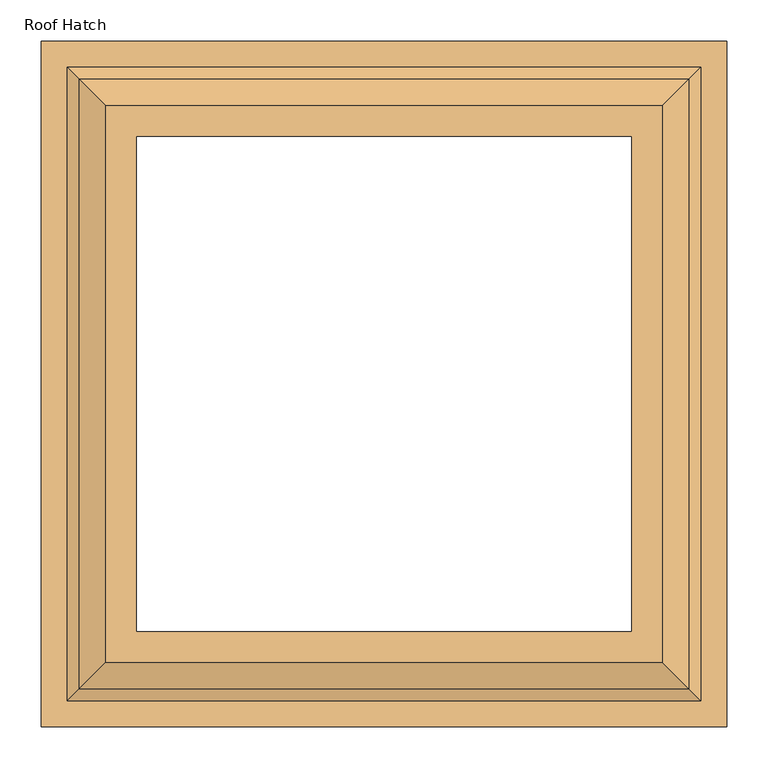
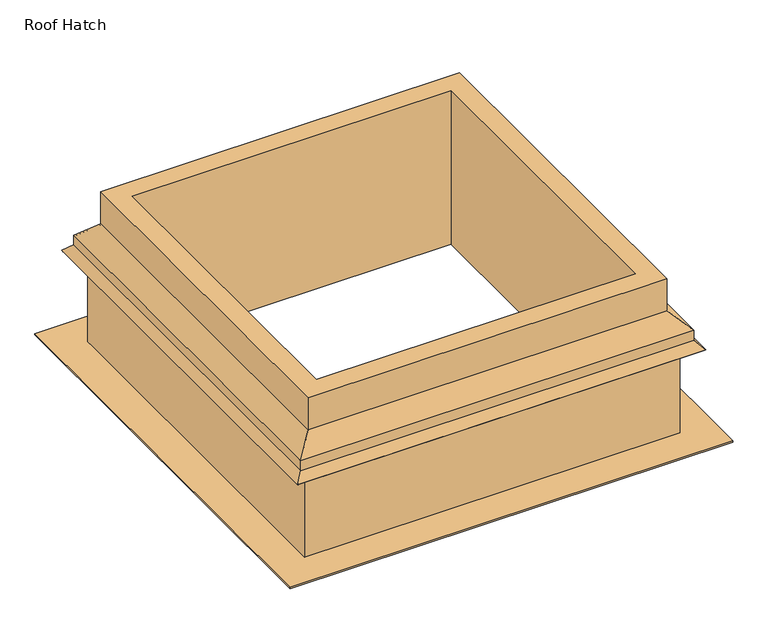
"""IFC4 building model written with IfcOpenShell, lengths in millimetres: door geometry, Alçap_o : Roof Hatch."""

from ifc_helpers import new_model, si_unit, origin, place, context, project, spatial, faceted_brep, source, transform, mapped, element, save


def roof_hatch_26298362(model_context):
    return source(origin(), model_context, "Body", "Brep", [
        faceted_brep([(119.78125, 353.18125, 2.38125), (119.78125, 353.18125, 224.63125), (119.78125, -353.18125, 224.63125), (119.78125, -353.18125, 2.38125), (68.98125, 302.38125, 230.98125), (68.98125, 302.38125, 2.38125), (68.98125, -302.38125, 2.38125), (68.98125, -302.38125, 230.98125), (-586.58125, -353.18125, 224.63125), (-586.58125, -353.18125, 2.38125), (-535.78125, -302.38125, 2.38125), (-535.78125, -302.38125, 230.98125), (-586.58125, 353.18125, 224.63125), (-586.58125, 353.18125, 2.38125), (-535.78125, 302.38125, 2.38125), (-535.78125, 302.38125, 230.98125), (113.43125, 346.83125, 230.98125), (-580.23125, 346.83125, 230.98125), (-580.23125, -346.83125, 230.98125), (113.43125, -346.83125, 230.98125)], [[[0, 1, 2, 3]], [[4, 5, 6, 7]], [[3, 2, 8, 9]], [[7, 6, 10, 11]], [[9, 8, 12, 13]], [[11, 10, 14, 15]], [[16, 17, 18, 19], [7, 11, 15, 4]], [[13, 12, 1, 0]], [[3, 9, 13, 0], [5, 14, 10, 6]], [[15, 14, 5, 4]], [[1, 16, 19, 2]], [[2, 19, 18, 8]], [[8, 18, 17, 12]], [[12, 17, 16, 1]]]),
        faceted_brep([(66.6, 300.0, 304.8), (66.6, 300.0, 0.0), (66.6, -300.0, 0.0), (66.6, -300.0, 304.8), (104.303125, 337.703125, 241.3), (104.303125, 337.703125, 304.8), (104.303125, -337.703125, 304.8), (104.303125, -337.703125, 241.3), (136.45, 369.85, 190.5), (136.45, 369.85, 210.1272727), (136.45, -369.85, 210.1272727), (136.45, -369.85, 190.5), (151.134375, 384.534375, 175.815625), (151.134375, -384.534375, 175.815625), (149.450577, 382.850577, 174.131827), (149.450577, -382.850577, 174.131827), (134.06875, 367.46875, 189.513654), (134.06875, -367.46875, 189.513654), (134.06875, 367.46875, 209.1193993), (134.06875, -367.46875, 209.1193993), (101.921875, 335.321875, 302.41875), (101.921875, 335.321875, 240.2921266), (101.921875, -335.321875, 240.2921266), (101.921875, -335.321875, 302.41875), (68.98125, 302.38125, 2.38125), (68.98125, 302.38125, 302.41875), (68.98125, -302.38125, 302.41875), (68.98125, -302.38125, 2.38125), (182.884375, 416.284375, 0.0), (182.884375, 416.284375, 2.38125), (182.884375, -416.284375, 2.38125), (182.884375, -416.284375, 0.0), (-533.4, -300.0, 0.0), (-533.4, -300.0, 304.8), (-571.103125, -337.703125, 304.8), (-571.103125, -337.703125, 241.3), (-603.25, -369.85, 210.1272727), (-603.25, -369.85, 190.5), (-617.934375, -384.534375, 175.815625), (-616.250577, -382.850577, 174.131827), (-600.86875, -367.46875, 189.513654), (-600.86875, -367.46875, 209.1193993), (-568.721875, -335.321875, 240.2921266), (-568.721875, -335.321875, 302.41875), (-535.78125, -302.38125, 302.41875), (-535.78125, -302.38125, 2.38125), (-649.684375, -416.284375, 2.38125), (-649.684375, -416.284375, 0.0), (-533.4, 300.0, 0.0), (-533.4, 300.0, 304.8), (-571.103125, 337.703125, 304.8), (-571.103125, 337.703125, 241.3), (-603.25, 369.85, 210.1272727), (-603.25, 369.85, 190.5), (-617.934375, 384.534375, 175.815625), (-616.250577, 382.850577, 174.131827), (-600.86875, 367.46875, 189.513654), (-600.86875, 367.46875, 209.1193993), (-568.721875, 335.321875, 240.2921266), (-568.721875, 335.321875, 302.41875), (-535.78125, 302.38125, 302.41875), (-535.78125, 302.38125, 2.38125), (-649.684375, 416.284375, 2.38125), (-649.684375, 416.284375, 0.0)], [[[0, 1, 2, 3]], [[4, 5, 6, 7]], [[8, 9, 10, 11]], [[12, 8, 11, 13]], [[14, 12, 13, 15]], [[16, 14, 15, 17]], [[18, 16, 17, 19]], [[20, 21, 22, 23]], [[24, 25, 26, 27]], [[28, 29, 30, 31]], [[3, 2, 32, 33]], [[7, 6, 34, 35]], [[11, 10, 36, 37]], [[13, 11, 37, 38]], [[15, 13, 38, 39]], [[17, 15, 39, 40]], [[19, 17, 40, 41]], [[23, 22, 42, 43]], [[27, 26, 44, 45]], [[31, 30, 46, 47]], [[33, 32, 48, 49]], [[35, 34, 50, 51]], [[37, 36, 52, 53]], [[38, 37, 53, 54]], [[39, 38, 54, 55]], [[40, 39, 55, 56]], [[41, 40, 56, 57]], [[43, 42, 58, 59]], [[45, 44, 60, 61]], [[47, 46, 62, 63]], [[49, 48, 1, 0]], [[5, 50, 34, 6], [3, 33, 49, 0]], [[51, 50, 5, 4]], [[53, 52, 9, 8]], [[54, 53, 8, 12]], [[55, 54, 12, 14]], [[56, 55, 14, 16]], [[57, 56, 16, 18]], [[59, 58, 21, 20]], [[23, 43, 59, 20], [25, 60, 44, 26]], [[61, 60, 25, 24]], [[29, 62, 46, 30], [27, 45, 61, 24]], [[63, 62, 29, 28]], [[31, 47, 63, 28], [1, 48, 32, 2]], [[9, 4, 7, 10]], [[21, 18, 19, 22]], [[10, 7, 35, 36]], [[22, 19, 41, 42]], [[36, 35, 51, 52]], [[42, 41, 57, 58]], [[52, 51, 4, 9]], [[58, 57, 18, 21]]]),
    ])


if __name__ == "__main__":
    model = new_model("IFC4")
    model_context = context("Model", 3, world=origin())
    ifc_project = project(units=[si_unit("LENGTHUNIT", "METRE", prefix="MILLI")], contexts=[model_context])
    site = spatial("IfcSite", under=ifc_project)
    building = spatial("IfcBuilding", under=site)
    placement = place(None, origin())
    roof_hatch_shape = roof_hatch_26298362(model_context)
    element("IfcDoor", 1, ObjectType="Alçap_o : Roof Hatch", at=placement, inside=building, context=model_context, shape_type="MappedRepresentation", body=[
        mapped(roof_hatch_shape, transform((0.0, 0.0, 0.0), x_axis=(1.0, 0.0, 0.0), y_axis=(0.0, 1.0, 0.0), z_axis=(0.0, 0.0, 1.0))),
    ])
    save(model, "model.ifc")

# Revit data of these elements
# Project information
#   Data de emissão do projeto = "Data de emissão"
#   Status do projeto = "Status do projeto"
#   Nome do cliente = "Proprietário"
#   Endereço do projeto = "RUA A - BLOCO A"
#   Nome do projeto = "CURSO REVIT PLANTA HUMANIZADA"
#   Número do projeto = "Número do projeto"
# Type "Alçap_o : Roof Hatch"
#   Type Mark = "P73"
#   Warranty = ""
#   URL Product = "http://www.bilco.com/foundations/store/shopdetail.asp?product=1S-1"
#   URL = "http://www.bilco.com/"
#   Analytic Construction = "<Nenhum>"
#   Release Date = ""
#   Observations = ""
#   Model = "Type S Roof Hatch"
#   Manufacturer = "Bilco"
#   Line = ""
#   Installation = ""
#   Industry Standards = ""
#   Designer = ""
#   Description = "Roof Hatch"
#   Date Maintenance = ""
#   Date Installation = ""
#   Customer Service Contact = ""
#   Created by = "Contino"
#   Certification = ""
#   Assembly Code = "B2030900"
#   Appoved by = "Contino"
#   Width = 0.600 m
#   Weight = 0
#   Rough Width = 0.6508 m
#   Rough Height = 0.6508 m
#   Length = 0.600 m
#   Height = 0.319881 m
#   Default Elevation = 1.2192 m
#   Cover Width = 0.73335 m
#   Cover Opening = 90.00°
#   Cover Length = 0.7016 m
#   Hatch Open [instance default] = yes
#   Hardware = Stainless Steel-Bilco-Sand Blast Finish-304
#   Gasket = Plastic-Bilco-Rubber Black
#   Frame = Stainless Steel-Bilco-Sand Blast Finish-304
#   Finish = Galvanized Steel - Bilco - Red Oxide Primer Finish
#   Fiberboard Insulation = Insulation-Bilco-Rigid Insulation
#   Dome = Plastic-Bilco-Polycarbonate
#   Cover = Galvanized Steel-Bilco-Red Oxide Primer Finish
#   Function = (empty or 0)
# Element 1 (IfcDoor, "Alçap_o : Roof Hatch")
#   Hatch Open = no
#   Materials on its faces: "Stainless Steel-Bilco-Sand Blast Finish-304", "Insulation-Bilco-Rigid Insulation"
# Materials
#   "Stainless Steel-Bilco-Sand Blast Finish-304": class "Metal", colour RGB 189 187 185, transparency 0, Manufacturer = "Add Manufacturer Name", URL = "Add Manufacturer URL", Cost = 0
#   "Plastic-Bilco-Rubber Black": class "Plastic", colour RGB 63 63 63, transparency 0, Manufacturer = "Add Manufacturer Name", URL = "Add Manufacturer URL", Cost = 0
#   "Galvanized Steel - Bilco - Red Oxide Primer Finish": class "Metal", colour RGB 160 81 45, transparency 0, Manufacturer = "Add Manufacturer Name", URL = "Add Manufacturer URL", Cost = 0
#   "Insulation-Bilco-Rigid Insulation": class "Miscellaneous", colour RGB 182 181 179, transparency 0
#   "Plastic-Bilco-Polycarbonate": class "Plastic", colour RGB 165 165 165, transparency 0.46, Cost = 0
#   "Galvanized Steel-Bilco-Red Oxide Primer Finish": class "Paint", colour RGB 160 81 45, transparency 0, Manufacturer = "Add Manufacturer Name", URL = "Add Manufacturer URL", Cost = 0
